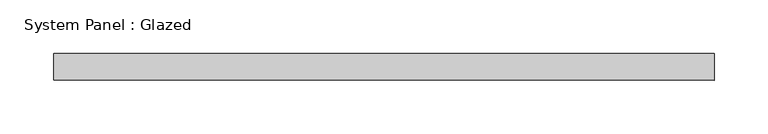
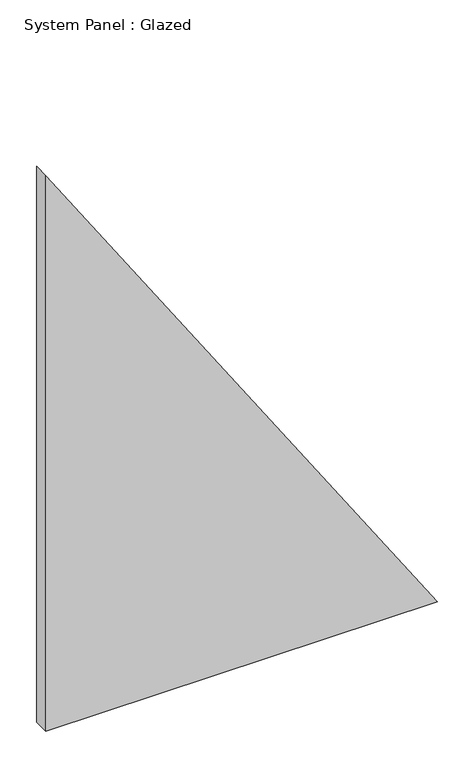
"""IFC4 building model written with IfcOpenShell, lengths in millimetres: plate geometry, System Panel : Glazed."""

from ifc_helpers import new_model, si_unit, frame, origin, place, context, project, spatial, polyline, outline, extrude, source, transform, mapped, element, save


def system_panel_glazed_162ceefa(model_context):
    return source(origin(), model_context, "Body", "SweptSolid", [
        extrude(outline(polyline([(0.0, -308.2508456), (0.0, 308.2508456), (924.6254194, -308.2508456), (0.0, -308.2508456)])), frame((0.0, 24.5, 0.0), z_axis=(0.0, 1.0, 0.0), x_axis=(0.0, 0.0, 1.0)), (0.0, 0.0, 1.0), 25.0),
    ])


if __name__ == "__main__":
    model = new_model("IFC4")
    model_context = context("Model", 3, world=origin())
    ifc_project = project(units=[si_unit("LENGTHUNIT", "METRE", prefix="MILLI")], contexts=[model_context])
    site = spatial("IfcSite", under=ifc_project)
    building = spatial("IfcBuilding", under=site)
    placement = place(None, origin())
    system_panel_glazed_shape = system_panel_glazed_162ceefa(model_context)
    element("IfcPlate", 1, ObjectType="System Panel : Glazed", at=placement, inside=building, context=model_context, shape_type="MappedRepresentation", body=[
        mapped(system_panel_glazed_shape, transform((0.0, 0.0, 0.0), x_axis=(1.0, 0.0, 0.0), y_axis=(0.0, 1.0, 0.0), z_axis=(0.0, 0.0, 1.0))),
    ])
    save(model, "model.ifc")

# Revit data of these elements
# Type "System Panel : Glazed"
#   Keynote = "H11"
#   Construction Type Id = "GSP4R"
#   Analytic Construction = "1/8 in Pilkington single glazing"
#   Visual Light Transmittance = 0.9
#   Solar Heat Gain Coefficient = 0.86
#   Heat Transfer Coefficient (U) = 6.7069 W/(m²·K)
#   Define Thermal Properties by = 1
# Element 1 (IfcPlate, "System Panel : Glazed")
#   Materials on its faces: "Glass"
# Materials
#   "Glass": class "Glass", colour RGB 0 128 192, transparency 0.9, Description = "Soda Lime Glass", Cost = 0
